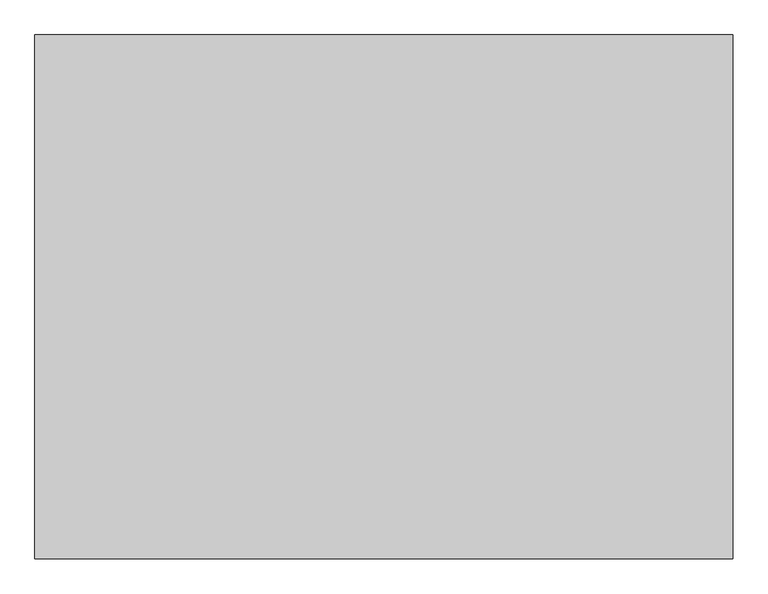
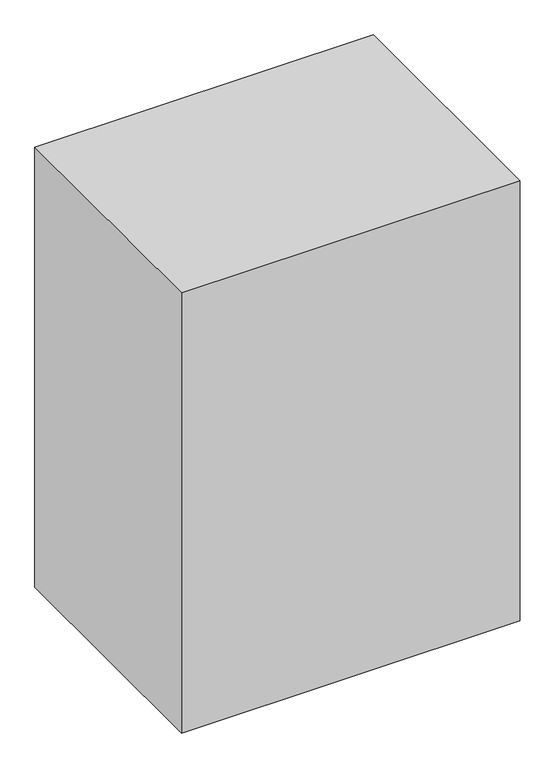
"""IFC4 building model written with IfcOpenShell, lengths in millimetres: proxy geometry, Space Planning Box_hec : Space Planning Box_hec."""

import ifcopenshell
import ifcopenshell.guid

model = None  # the IFC model being written
_history = None  # IfcOwnerHistory: only IFC2X3 demands one
_inside = {}  # id of a spatial element -> (the spatial element, [elements in it])
_under = {}  # id of a project, library or spatial element -> (it, [spatial elements below it])
_declared = {}  # id of a project -> (the project, [libraries it declares])
_typed = {}  # id of a type object -> (the type object, [elements of that type])
_made_of = {}  # id of a material, layer set ... -> (it, [elements and type objects made of it])


def new_model(schema):
    """Start an empty IFC model of exactly this schema.

    Asked for "IFC4X3", IfcOpenShell would pick the latest addendum, in which some entities
    have other attributes; the version numbers below select the first issue.
    IFC2X3 requires an IfcOwnerHistory on every rooted entity: one is made here for all.
    """
    global model, _history
    if schema == "IFC4X3":
        model = ifcopenshell.file(schema_version=(4, 3, 0, 0))
    else:
        model = ifcopenshell.file(schema=schema)
    _inside.clear()
    _under.clear()
    _declared.clear()
    _typed.clear()
    _made_of.clear()
    _history = None
    if model.schema == "IFC2X3":
        org = make("IfcOrganization", Name="unknown")
        user = make(
            "IfcPersonAndOrganization",
            ThePerson=make("IfcPerson", FamilyName="unknown"),
            TheOrganization=org,
        )
        app = make(
            "IfcApplication",
            ApplicationDeveloper=org,
            Version="unknown",
            ApplicationFullName="unknown",
            ApplicationIdentifier="unknown",
        )
        _history = make(
            "IfcOwnerHistory",
            OwningUser=user,
            OwningApplication=app,
            ChangeAction="ADDED",
            CreationDate=0,
        )
    return model


def make(cls, **values):
    """One entity of the class cls with the attributes given. An attribute that is None is left unset."""
    return model.create_entity(
        cls, **{name: value for name, value in values.items() if value is not None}
    )


def rooted(cls, **values):
    """An entity with a GlobalId (a new one), such as an element, a storey or a relation."""
    return make(cls, GlobalId=ifcopenshell.guid.new(), OwnerHistory=_history, **values)


def si_unit(unit_type, name, prefix=None):
    """IfcSIUnit, for example si_unit("LENGTHUNIT", "METRE", prefix="MILLI")."""
    return make("IfcSIUnit", UnitType=unit_type, Prefix=prefix, Name=name)


def assignment(units):
    """IfcUnitAssignment: the units of a project."""
    return None if units is None else make("IfcUnitAssignment", Units=units)


def point(xyz):
    """IfcCartesianPoint."""
    return None if xyz is None else make("IfcCartesianPoint", Coordinates=xyz)


def direction(xyz):
    """IfcDirection."""
    return None if xyz is None else make("IfcDirection", DirectionRatios=xyz)


def frame(location, z_axis=None, x_axis=None):
    """IfcAxis2Placement3D, a coordinate frame: its origin and axes. An axis left out is left unset."""
    return make(
        "IfcAxis2Placement3D",
        Location=point(location),
        Axis=direction(z_axis),
        RefDirection=direction(x_axis),
    )


def origin():
    """The frame at (0, 0, 0) with its axes left unset."""
    return frame((0.0, 0.0, 0.0))


def origin_with_axes():
    """The frame at (0, 0, 0) with the z axis (0, 0, 1) and the x axis (1, 0, 0) written out."""
    return frame((0.0, 0.0, 0.0), z_axis=(0.0, 0.0, 1.0), x_axis=(1.0, 0.0, 0.0))


def place(relative_to, where):
    """IfcLocalPlacement: puts the frame where relative to a parent placement (None: the world)."""
    return make(
        "IfcLocalPlacement", PlacementRelTo=relative_to, RelativePlacement=where
    )


def context(
    kind, dimensions, precision=None, world=None, true_north=None, identifier=None
):
    """IfcGeometricRepresentationContext, for example the 3D "Model" context."""
    return make(
        "IfcGeometricRepresentationContext",
        ContextIdentifier=identifier,
        ContextType=kind,
        CoordinateSpaceDimension=dimensions,
        Precision=precision,
        WorldCoordinateSystem=world,
        TrueNorth=true_north,
    )


def project(units=None, contexts=None):
    """IfcProject with its units and contexts."""
    return rooted(
        "IfcProject",
        Name="project",
        RepresentationContexts=contexts,
        UnitsInContext=assignment(units),
    )


def spatial(cls, under=None, at=None, **own):
    """A site, building, storey or space (cls), placed at a placement, below another one or the project."""
    s = rooted(cls, ObjectPlacement=at, **own)
    if under is not None:
        _under.setdefault(under.id(), (under, []))[1].append(s)
    return s


def polyline(points):
    """IfcPolyline through the points."""
    return make("IfcPolyline", Points=[point(p) for p in points])


def outline(outer, holes=None, kind="AREA"):
    """IfcArbitraryClosedProfileDef: a profile drawn as a closed curve; with holes, ...WithVoids."""
    if holes is None:
        return make("IfcArbitraryClosedProfileDef", ProfileType=kind, OuterCurve=outer)
    return make(
        "IfcArbitraryProfileDefWithVoids",
        ProfileType=kind,
        OuterCurve=outer,
        InnerCurves=holes,
    )


def extrude(swept, where, along, depth):
    """IfcExtrudedAreaSolid: the profile swept, set in the frame where, extruded along a direction by depth."""
    return make(
        "IfcExtrudedAreaSolid",
        SweptArea=swept,
        Position=where,
        ExtrudedDirection=direction(along),
        Depth=depth,
    )


def shape(context_of_items, identifier, shape_type, items):
    """IfcShapeRepresentation: the items that make up one representation, for example the "Body"."""
    return make(
        "IfcShapeRepresentation",
        ContextOfItems=context_of_items,
        RepresentationIdentifier=identifier,
        RepresentationType=shape_type,
        Items=items,
    )


def source(mapping_origin, context_of_items, identifier, shape_type, items):
    """IfcRepresentationMap: a shape defined once, which mapped items show again and again."""
    return make(
        "IfcRepresentationMap",
        MappingOrigin=mapping_origin,
        MappedRepresentation=shape(context_of_items, identifier, shape_type, items),
    )


def transform(
    local_origin,
    x_axis=None,
    y_axis=None,
    z_axis=None,
    scale=None,
    scale2=None,
    scale3=None,
    uniform=True,
):
    """IfcCartesianTransformationOperator3D, or its non-uniform kind. x_axis, y_axis, z_axis: its Axis1, 2, 3."""
    if uniform:
        return make(
            "IfcCartesianTransformationOperator3D",
            Axis1=direction(x_axis),
            Axis2=direction(y_axis),
            LocalOrigin=point(local_origin),
            Scale=scale,
            Axis3=direction(z_axis),
        )
    return make(
        "IfcCartesianTransformationOperator3DnonUniform",
        Axis1=direction(x_axis),
        Axis2=direction(y_axis),
        LocalOrigin=point(local_origin),
        Scale=scale,
        Axis3=direction(z_axis),
        Scale2=scale2,
        Scale3=scale3,
    )


def mapped(mapping_source, mapping_target):
    """IfcMappedItem: shows the shape of a source again, moved by a transform."""
    return make(
        "IfcMappedItem", MappingSource=mapping_source, MappingTarget=mapping_target
    )


def made_of(thing, what):
    """Note that an element or type object is made of a material, layer set ...; save() writes the relation."""
    if what is not None:
        _made_of.setdefault(what.id(), (what, []))[1].append(thing)
    return thing


def element(
    cls,
    number,
    at=None,
    inside=None,
    cuts=None,
    type_object=None,
    material=None,
    context=None,
    identifier="Body",
    shape_type=None,
    held_by="IfcProductDefinitionShape",
    body=None,
    shapes=None,
    **own,
):
    """One element of the class cls, such as IfcWall. Its Tag is "e" and its number.

    at: its placement. inside: the storey or other place that contains it. cuts: it is an
    opening in that element (IfcRelVoidsElement). A single representation is given by context,
    identifier, shape_type and body (its items); several are given by shapes. held_by: the class
    of the entity that holds the representations. save() writes the other relations.
    """
    e = rooted(cls, Tag="e%d" % number, ObjectPlacement=at, **own)
    if body is not None:
        shapes = [shape(context, identifier, shape_type, body)]
    if shapes is not None:
        e.Representation = make(held_by, Representations=shapes)
    if inside is not None:
        _inside.setdefault(inside.id(), (inside, []))[1].append(e)
    if cuts is not None:
        rooted(
            "IfcRelVoidsElement", RelatingBuildingElement=cuts, RelatedOpeningElement=e
        )
    if type_object is not None:
        _typed.setdefault(type_object.id(), (type_object, []))[1].append(e)
    return made_of(e, material)


def aggregate(whole, parts):
    """IfcRelAggregates: a whole, such as a stair, and the parts it consists of."""
    return rooted("IfcRelAggregates", RelatingObject=whole, RelatedObjects=parts)


def save(model, path):
    """Write the relations noted so far, then the file.

    IfcRelAggregates (storeys below a building ...), IfcRelContainedInSpatialStructure (elements
    in a storey), IfcRelDefinesByType, IfcRelAssociatesMaterial and IfcRelDeclares: one each for
    every whole, place, type object, material and project.
    """
    for whole, parts in _under.values():
        aggregate(whole, parts)
    for where, things in _inside.values():
        rooted(
            "IfcRelContainedInSpatialStructure",
            RelatedElements=things,
            RelatingStructure=where,
        )
    for kind, things in _typed.values():
        rooted("IfcRelDefinesByType", RelatedObjects=things, RelatingType=kind)
    for what, things in _made_of.values():
        rooted("IfcRelAssociatesMaterial", RelatedObjects=things, RelatingMaterial=what)
    for by, libraries in _declared.values():
        rooted("IfcRelDeclares", RelatingContext=by, RelatedDefinitions=libraries)
    model.write(path)


def generic_models_626d8198(model_context):
    return source(origin(), model_context, "Body", "SweptSolid", [
        extrude(outline(polyline([(2000.0, 1500.0), (2000.0, -1500.0), (-2000.0, -1500.0), (-2000.0, 1500.0), (2000.0, 1500.0)])), origin_with_axes(), (0.0, 0.0, 1.0), 5500.0),
    ])


if __name__ == "__main__":
    model = new_model("IFC4")
    model_context = context("Model", 3, world=origin())
    ifc_project = project(units=[si_unit("LENGTHUNIT", "METRE", prefix="MILLI")], contexts=[model_context])
    site = spatial("IfcSite", under=ifc_project)
    building = spatial("IfcBuilding", under=site)
    placement = place(None, origin())
    generic_models_shape = generic_models_626d8198(model_context)
    element("IfcBuildingElementProxy", 1, Name="Space Planning Box_hec : Space Planning Box_hec", ObjectType="Space Planning Box_hec : Space Planning Box_hec", at=placement, inside=building, context=model_context, shape_type="MappedRepresentation", body=[
        mapped(generic_models_shape, transform((0.0, 0.0, 0.0), x_axis=(1.0, 0.0, 0.0), y_axis=(0.0, 1.0, 0.0), z_axis=(0.0, 0.0, 1.0))),
    ])
    save(model, "model.ifc")

# Revit data of these elements
# Type "Space Planning Box_hec : Space Planning Box_hec"
#   Type Comments = "..."
#   Room Name [instance default] = "?"
#   Interior Finish [instance default] = ""
#   Exterior Finish [instance default] = ""
#   Department [instance default] = ""
#   Assembly Code = "..."
#   ceiling height [instance default] = 0
#   Width [instance default] = 1524 mm
#   Program Area [instance default] = 0.00 m²
#   Length [instance default] = 1524 mm
#   Height [instance default] = 1524 mm
#   Area [instance default] = 2.32258 m²
#   Fill Color [instance default] = Cyan
#   Default Elevation = 0
# Element 1 (IfcBuildingElementProxy, "Space Planning Box_hec : Space Planning Box_hec")
#   Room Name = "Elevator"
#   Exterior Finish = "N/A..N/A,,EW2..N/A..N/A"
#   Department = "PATHV2"
#   Width = 4000 mm
#   Program Area = 12.00 m²
#   Length = 3000 mm
#   Height = 5500 mm
#   Area = 12.00 m²
#   Fill Color = Blue
#   Materials on its faces: "Blue"
# Materials
#   "Cyan": class "Generic", colour RGB 0 255 255, transparency 0.2, Cost = 0
#   "Blue": class "Generic", colour RGB 0 0 255, transparency 0.2, Cost = 0
